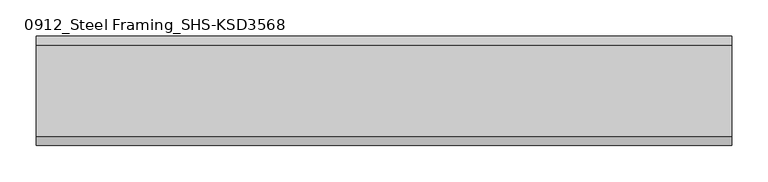
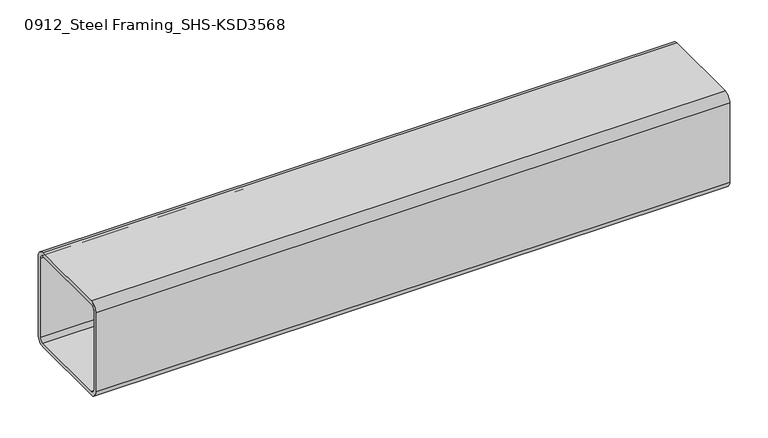
"""IFC4 building model written with IfcOpenShell, lengths in millimetres: beam geometry, 0912_Steel Framing_SHS-KSD3568 : H_SB_ASB_SHS-150x150x6."""

from ifc_helpers import new_model, si_unit, point, frame, frame_2d, origin, place, context, project, spatial, polyline, circle_curve, trimmed, segment, composite_curve, outline, extrude, source, transform, mapped, element, save


def beam_0912_steel_framing_shs_ksd3568_73b27394(model_context):
    return source(origin(), model_context, "Body", "SweptSolid", [
        extrude(outline(composite_curve([segment(polyline([(75.0, 63.0), (75.0, -63.0)]), True, "CONTINUOUS"), segment(trimmed(circle_curve(frame_2d((63.0, -63.0)), 12.0), [point((75.0, -63.0))], [point((63.0, -75.0))], False, "CARTESIAN"), True, "CONTINUOUS"), segment(polyline([(63.0, -75.0), (-63.0, -75.0)]), True, "CONTINUOUS"), segment(trimmed(circle_curve(frame_2d((-63.0, -63.0)), 12.0), [point((-63.0, -75.0))], [point((-75.0, -63.0))], False, "CARTESIAN"), True, "CONTINUOUS"), segment(polyline([(-75.0, -63.0), (-75.0, 63.0)]), True, "CONTINUOUS"), segment(trimmed(circle_curve(frame_2d((-63.0, 63.0)), 12.0), [point((-75.0, 63.0))], [point((-63.0, 75.0))], False, "CARTESIAN"), True, "CONTINUOUS"), segment(polyline([(-63.0, 75.0), (63.0, 75.0)]), True, "CONTINUOUS"), segment(trimmed(circle_curve(frame_2d((63.0, 63.0)), 12.0), [point((63.0, 75.0))], [point((75.0, 63.0))], False, "CARTESIAN"), True, "CONTINUOUS")], self_intersect=False), holes=[composite_curve([segment(trimmed(circle_curve(frame_2d((-63.0, 63.0)), 6.0), [point((-63.0, 69.0))], [point((-69.0, 63.0))], True, "CARTESIAN"), True, "CONTINUOUS"), segment(polyline([(-69.0, 63.0), (-69.0, -63.0)]), True, "CONTINUOUS"), segment(trimmed(circle_curve(frame_2d((-63.0, -63.0)), 6.0), [point((-69.0, -63.0))], [point((-63.0, -69.0))], True, "CARTESIAN"), True, "CONTINUOUS"), segment(polyline([(-63.0, -69.0), (63.0, -69.0)]), True, "CONTINUOUS"), segment(trimmed(circle_curve(frame_2d((63.0, -63.0)), 6.0), [point((63.0, -69.0))], [point((69.0, -63.0))], True, "CARTESIAN"), True, "CONTINUOUS"), segment(polyline([(69.0, -63.0), (69.0, 63.0)]), True, "CONTINUOUS"), segment(trimmed(circle_curve(frame_2d((63.0, 63.0)), 6.0), [point((69.0, 63.0))], [point((63.0, 69.0))], True, "CARTESIAN"), True, "CONTINUOUS"), segment(polyline([(63.0, 69.0), (-63.0, 69.0)]), True, "CONTINUOUS")], self_intersect=False)]), frame((-477.5002564, 0.0, 0.0), z_axis=(1.0, 0.0, 0.0), x_axis=(0.0, 1.0, 0.0)), (0.0, 0.0, 1.0), 955.0005128),
    ])


if __name__ == "__main__":
    model = new_model("IFC4")
    model_context = context("Model", 3, world=origin())
    ifc_project = project(units=[si_unit("LENGTHUNIT", "METRE", prefix="MILLI")], contexts=[model_context])
    site = spatial("IfcSite", under=ifc_project)
    building = spatial("IfcBuilding", under=site)
    placement = place(None, origin())
    beam_0912_steel_framing_shs_ksd3568_shape = beam_0912_steel_framing_shs_ksd3568_73b27394(model_context)
    element("IfcBeam", 1, ObjectType="0912_Steel Framing_SHS-KSD3568 : H_SB_ASB_SHS-150x150x6", at=placement, inside=building, context=model_context, shape_type="MappedRepresentation", body=[
        mapped(beam_0912_steel_framing_shs_ksd3568_shape, transform((0.0, 0.0, 0.0), x_axis=(1.0, 0.0, 0.0), y_axis=(0.0, 1.0, 0.0), z_axis=(0.0, 0.0, 1.0))),
    ])
    save(model, "model.ifc")

# Revit data of these elements
# Type "0912_Steel Framing_SHS-KSD3568 : H_SB_ASB_SHS-150x150x6"
#   H_WM Code_1 = "S01AA002-00001 | Main Steel Structure Fabrication Work | Shelter/Building | Medium Steel - Standard (90KG/M>Weight≥30KG/M) | Material: (   )"
#   H_WM Code_2 = "S03AA028-00001 | Main Steel Structure Erection Work | Shelter/Building | Medium Steel (90KG/M>Weight≥30KG/M) | Material: (   )"
#   H_WM Code_3 = "S01AA010-00001 | Main Steel Structure Fabrication Work | Shelter/Building | Steel Painting/Coating | for Non-Fireproofed Steel Surface, Surface Preparation, Primer, Second & Final Coat | Material: (   )"
#   H_Q'ty Cal Type Tag = "SB-Q2"
#   Perimeter = 0.60 m²/m
#   Nominal Weight = 26.40 kgf/m
#   Length [instance default] = 1.0000 m
#   b = 0.1500 m
#   h = 0.1500 m
#   tr = 0.0120 m
#   t = 0.0060 m
#   A = 28.36 m²
#   Structural Material [instance default] = Steel, 45-345
# Element 1 (IfcBeam, "0912_Steel Framing_SHS-KSD3568 : H_SB_ASB_SHS-150x150x6")
#   Structural Material = none
# Materials
#   "Steel, 45-345": class "Metal", colour RGB 189 187 185, transparency 0, Description = "Steel 345 MPa", Cost = 0
